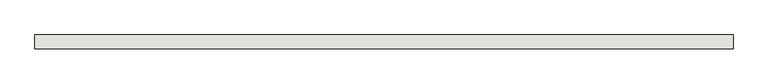
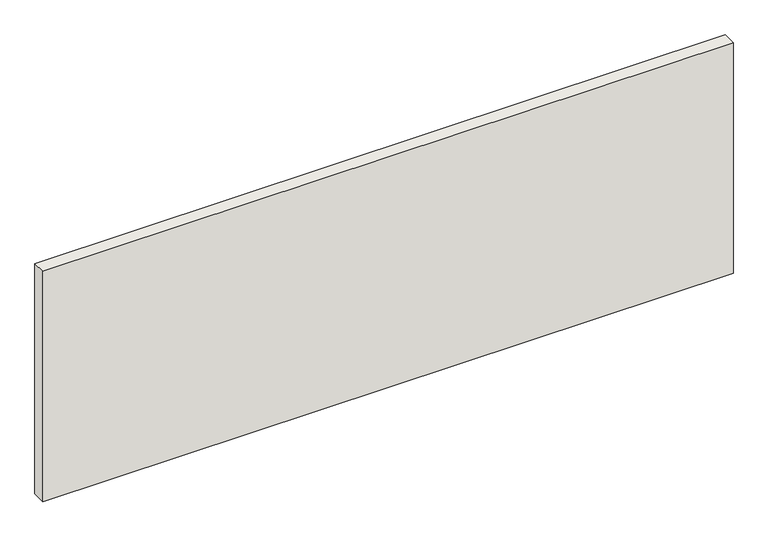
"""IFC4 building model written with IfcOpenShell, lengths in millimetres: wall geometry, Holzwand."""

from ifc_helpers import new_model, si_unit, origin, origin_with_axes, place, context, project, spatial, polyline, outline, extrude, source, transform, mapped, element, save


def wall_ca4d3ae7(model_context):
    return source(origin(), model_context, "Body", "SweptSolid", [
        extrude(outline(polyline([(0.0, 50.0), (2550.0, 50.0), (2550.0, 0.0), (0.0, 0.0), (0.0, 50.0)])), origin_with_axes(), (0.0, 0.0, 1.0), 900.0),
    ])


if __name__ == "__main__":
    model = new_model("IFC4")
    model_context = context("Model", 3, world=origin())
    ifc_project = project(units=[si_unit("LENGTHUNIT", "METRE", prefix="MILLI")], contexts=[model_context])
    site = spatial("IfcSite", under=ifc_project)
    building = spatial("IfcBuilding", under=site)
    placement = place(None, origin())
    wall_shape = wall_ca4d3ae7(model_context)
    element("IfcWall", 1, ObjectType="Holzwand", at=placement, inside=building, context=model_context, shape_type="MappedRepresentation", body=[
        mapped(wall_shape, transform((0.0, 0.0, 0.0), x_axis=(1.0, 0.0, 0.0), y_axis=(0.0, 1.0, 0.0), z_axis=(0.0, 0.0, 1.0))),
    ])
    save(model, "model.ifc")

# Revit data of these elements
# Element 1 (IfcWall, "Holzwand")
#   Materials on its faces: "holzschalung"
# Materials
#   "holzschalung": class "Unassigned", colour RGB 128 128 128, transparency 0
